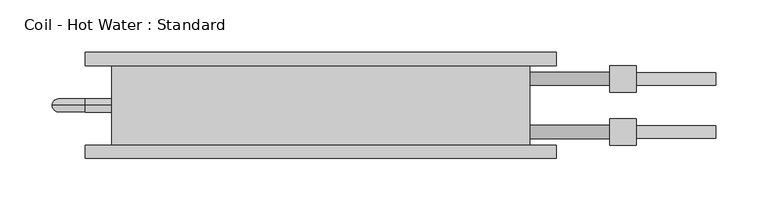
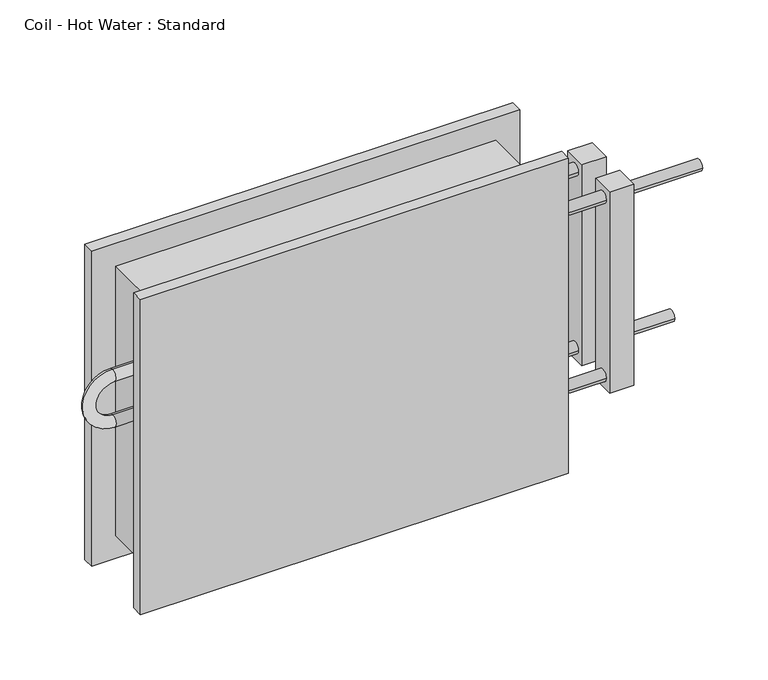
"""IFC4 building model written with IfcOpenShell, lengths in millimetres: proxy geometry, Coil - Hot Water : Standard."""

from ifc_helpers import new_model, si_unit, point, frame, origin, place, context, project, spatial, circle_curve, ellipse_curve, trimmed, source, transform, mapped, element, save
from ifc_brep_helpers import plane_surface, cylinder_surface, revolved_surface, advanced_brep


def coil_hot_water_standard_57d6a269(model_context):
    return source(origin(), model_context, "Body", "AdvancedBrep", [
        advanced_brep(
        [(-200.0, 76.2, 300.0), (-200.0, 0.0, 300.0), (200.0, 0.0, 300.0), (200.0, 76.2, 300.0), (200.0, 76.2, 0.0), (200.0, 0.0, 0.0), (-200.0, 0.0, 0.0), (-200.0, 76.2, 0.0), (-200.0, 38.1, 217.45), (-200.0, 38.1, 204.75), (-200.0, 38.1, 166.65), (-200.0, 38.1, 153.95), (200.0, 57.15, 249.2), (200.0, 69.85, 249.2), (200.0, 6.35, 50.8), (200.0, 19.05, 50.8), (200.0, 6.35, 249.2), (200.0, 19.05, 249.2), (200.0, 57.15, 50.8), (200.0, 69.85, 50.8), (225.4, 76.2, 325.4), (-225.4, 76.2, 325.4), (-225.4, 76.2, -25.4), (225.4, 76.2, -25.4), (225.4, 88.9, 325.4), (225.4, 88.9, -25.4), (-225.4, 88.9, -25.4), (-225.4, 88.9, 325.4), (377.8, 57.5, 50.8), (377.8, 69.5, 50.8), (377.8, 6.7, 249.2), (377.8, 18.7, 249.2), (301.6, 57.5, 50.8), (301.6, 69.5, 50.8), (301.6, 6.7, 249.2), (301.6, 18.7, 249.2), (225.4, -12.7, 325.4), (-225.4, -12.7, 325.4), (-225.4, -12.7, -25.4), (225.4, -12.7, -25.4), (225.4, 0.0, 325.4), (225.4, 0.0, -25.4), (-225.4, 0.0, -25.4), (-225.4, 0.0, 325.4), (-225.4, 38.1, 217.45), (-225.4, 38.1, 204.75), (-225.4, 38.1, 153.95), (-225.4, 38.1, 166.65), (276.2, 57.15, 249.2), (276.2, 69.85, 249.2), (276.2, 6.35, 50.8), (276.2, 19.05, 50.8), (276.2, 6.35, 249.2), (276.2, 19.05, 249.2), (276.2, 57.15, 50.8), (276.2, 69.85, 50.8), (301.6, 50.8, 261.9), (301.6, 50.8, 38.1), (301.6, 76.2, 38.1), (301.6, 76.2, 261.9), (301.6, 0.0, 261.9), (301.6, 0.0, 38.1), (301.6, 25.4, 38.1), (301.6, 25.4, 261.9), (276.2, 50.8, 261.9), (276.2, 76.2, 261.9), (276.2, 76.2, 38.1), (276.2, 50.8, 38.1), (276.2, 0.0, 261.9), (276.2, 25.4, 261.9), (276.2, 25.4, 38.1), (276.2, 0.0, 38.1)],
        [
            (0, 1),
            (1, 2),
            (2, 3),
            (3, 0),
            (4, 5),
            (5, 6),
            (6, 7),
            (7, 4),
            (0, 7),
            (6, 1),
            (8, 9, circle_curve(frame((-200.0, 38.1, 211.1), z_axis=(1.0, 0.0, 0.0), x_axis=(0.0, 0.0, -1.0)), 6.35)),
            (9, 8, circle_curve(frame((-200.0, 38.1, 211.1), z_axis=(1.0, 0.0, 0.0), x_axis=(0.0, 0.0, -1.0)), 6.35)),
            (10, 11, circle_curve(frame((-200.0, 38.1, 160.3), z_axis=(1.0, 0.0, 0.0), x_axis=(0.0, 0.0, 1.0)), 6.35)),
            (11, 10, circle_curve(frame((-200.0, 38.1, 160.3), z_axis=(1.0, 0.0, 0.0), x_axis=(0.0, 0.0, 1.0)), 6.35)),
            (2, 5),
            (4, 3),
            (12, 13, circle_curve(frame((200.0, 63.5, 249.2), z_axis=(-1.0, 0.0, 0.0), x_axis=(0.0, 1.0, 0.0)), 6.35)),
            (13, 12, circle_curve(frame((200.0, 63.5, 249.2), z_axis=(-1.0, 0.0, 0.0), x_axis=(0.0, 1.0, 0.0)), 6.35)),
            (14, 15, circle_curve(frame((200.0, 12.7, 50.8), z_axis=(-1.0, 0.0, 0.0), x_axis=(0.0, 1.0, 0.0)), 6.35)),
            (15, 14, circle_curve(frame((200.0, 12.7, 50.8), z_axis=(-1.0, 0.0, 0.0), x_axis=(0.0, 1.0, 0.0)), 6.35)),
            (16, 17, circle_curve(frame((200.0, 12.7, 249.2), z_axis=(-1.0, 0.0, 0.0), x_axis=(0.0, 1.0, 0.0)), 6.35)),
            (17, 16, circle_curve(frame((200.0, 12.7, 249.2), z_axis=(-1.0, 0.0, 0.0), x_axis=(0.0, 1.0, 0.0)), 6.35)),
            (18, 19, circle_curve(frame((200.0, 63.5, 50.8), z_axis=(-1.0, 0.0, 0.0), x_axis=(0.0, 1.0, 0.0)), 6.35)),
            (19, 18, circle_curve(frame((200.0, 63.5, 50.8), z_axis=(-1.0, 0.0, 0.0), x_axis=(0.0, 1.0, 0.0)), 6.35)),
            (20, 21),
            (21, 22),
            (22, 23),
            (23, 20),
            (24, 25),
            (25, 26),
            (26, 27),
            (27, 24),
            (20, 24),
            (27, 21),
            (26, 22),
            (25, 23),
            (28, 29, circle_curve(frame((377.8, 63.5, 50.8), z_axis=(1.0, 0.0, 0.0), x_axis=(0.0, 1.0, 0.0)), 6.0)),
            (29, 28, circle_curve(frame((377.8, 63.5, 50.8), z_axis=(1.0, 0.0, 0.0), x_axis=(0.0, 1.0, 0.0)), 6.0)),
            (30, 31, circle_curve(frame((377.8, 12.7, 249.2), z_axis=(1.0, 0.0, 0.0), x_axis=(0.0, 1.0, 0.0)), 6.0)),
            (31, 30, circle_curve(frame((377.8, 12.7, 249.2), z_axis=(1.0, 0.0, 0.0), x_axis=(0.0, 1.0, 0.0)), 6.0)),
            (28, 32),
            (32, 33, circle_curve(frame((301.6, 63.5, 50.8), z_axis=(1.0, 0.0, 0.0), x_axis=(0.0, 1.0, 0.0)), 6.0)),
            (33, 29),
            (33, 32, circle_curve(frame((301.6, 63.5, 50.8), z_axis=(1.0, 0.0, 0.0), x_axis=(0.0, 1.0, 0.0)), 6.0)),
            (30, 34),
            (34, 35, circle_curve(frame((301.6, 12.7, 249.2), z_axis=(1.0, 0.0, 0.0), x_axis=(0.0, 1.0, 0.0)), 6.0)),
            (35, 31),
            (35, 34, circle_curve(frame((301.6, 12.7, 249.2), z_axis=(1.0, 0.0, 0.0), x_axis=(0.0, 1.0, 0.0)), 6.0)),
            (36, 37),
            (37, 38),
            (38, 39),
            (39, 36),
            (40, 41),
            (41, 42),
            (42, 43),
            (43, 40),
            (36, 40),
            (43, 37),
            (42, 38),
            (41, 39),
            (8, 44),
            (44, 45, circle_curve(frame((-225.4, 38.1, 211.1), z_axis=(1.0, 0.0, 0.0), x_axis=(0.0, 0.0, -1.0)), 6.35)),
            (45, 9),
            (45, 44, circle_curve(frame((-225.4, 38.1, 211.1), z_axis=(1.0, 0.0, 0.0), x_axis=(0.0, 0.0, -1.0)), 6.35)),
            (44, 46, circle_curve(frame((-225.4, 38.1, 185.7), z_axis=(0.0, -1.0, 0.0), x_axis=(0.0, 0.0, 1.0)), 31.75)),
            (46, 47, circle_curve(frame((-225.4, 38.1, 160.3), z_axis=(-1.0, 0.0, 0.0), x_axis=(0.0, 0.0, 1.0)), 6.35)),
            (47, 45, circle_curve(frame((-225.4, 38.1, 185.7), z_axis=(0.0, 1.0, 0.0), x_axis=(0.0, 0.0, 1.0)), 19.05)),
            (47, 46, circle_curve(frame((-225.4, 38.1, 160.3), z_axis=(-1.0, 0.0, 0.0), x_axis=(0.0, 0.0, 1.0)), 6.35)),
            (46, 11),
            (10, 47),
            (12, 48),
            (48, 49, circle_curve(frame((276.2, 63.5, 249.2), z_axis=(-1.0, 0.0, 0.0), x_axis=(0.0, 1.0, 0.0)), 6.35)),
            (49, 13),
            (49, 48, circle_curve(frame((276.2, 63.5, 249.2), z_axis=(-1.0, 0.0, 0.0), x_axis=(0.0, 1.0, 0.0)), 6.35)),
            (14, 50),
            (50, 51, circle_curve(frame((276.2, 12.7, 50.8), z_axis=(-1.0, 0.0, 0.0), x_axis=(0.0, 1.0, 0.0)), 6.35)),
            (51, 15),
            (51, 50, circle_curve(frame((276.2, 12.7, 50.8), z_axis=(-1.0, 0.0, 0.0), x_axis=(0.0, 1.0, 0.0)), 6.35)),
            (16, 52),
            (52, 53, circle_curve(frame((276.2, 12.7, 249.2), z_axis=(-1.0, 0.0, 0.0), x_axis=(0.0, 1.0, 0.0)), 6.35)),
            (53, 17),
            (53, 52, circle_curve(frame((276.2, 12.7, 249.2), z_axis=(-1.0, 0.0, 0.0), x_axis=(0.0, 1.0, 0.0)), 6.35)),
            (18, 54),
            (54, 55, circle_curve(frame((276.2, 63.5, 50.8), z_axis=(-1.0, 0.0, 0.0), x_axis=(0.0, 1.0, 0.0)), 6.35)),
            (55, 19),
            (55, 54, circle_curve(frame((276.2, 63.5, 50.8), z_axis=(-1.0, 0.0, 0.0), x_axis=(0.0, 1.0, 0.0)), 6.35)),
            (56, 57),
            (57, 58),
            (58, 59),
            (59, 56),
            (60, 61),
            (61, 62),
            (62, 63),
            (63, 60),
            (64, 65),
            (65, 66),
            (66, 67),
            (67, 64),
            (68, 69),
            (69, 70),
            (70, 71),
            (71, 68),
            (56, 64),
            (67, 57),
            (66, 58),
            (65, 59),
            (60, 68),
            (71, 61),
            (70, 62),
            (69, 63),
        ],
        [
            plane_surface(frame((-200.0, 76.2, 300.0), z_axis=(0.0, 0.0, 1.0), x_axis=(-1.0, 0.0, 0.0))),
            plane_surface(frame((-200.0, 76.2, 0.0), z_axis=(0.0, 0.0, -1.0), x_axis=(1.0, 0.0, 0.0))),
            plane_surface(frame((-200.0, 76.2, 300.0), z_axis=(-1.0, 0.0, 0.0), x_axis=(0.0, 0.0, -1.0))),
            plane_surface(frame((200.0, 0.0, 300.0), z_axis=(1.0, 0.0, 0.0), x_axis=(0.0, 0.0, -1.0))),
            plane_surface(frame((-225.4, 76.2, 325.4), z_axis=(0.0, -1.0, 0.0), x_axis=(-1.0, 0.0, 0.0))),
            plane_surface(frame((-225.4, 88.9, 325.4), z_axis=(0.0, 1.0, 0.0), x_axis=(1.0, 0.0, 0.0))),
            plane_surface(frame((225.4, 76.2, 325.4), z_axis=(0.0, 0.0, 1.0), x_axis=(0.0, 1.0, 0.0))),
            plane_surface(frame((-225.4, 76.2, 325.4), z_axis=(-1.0, 0.0, 0.0), x_axis=(0.0, 1.0, 0.0))),
            plane_surface(frame((-225.4, 76.2, -25.4), z_axis=(0.0, 0.0, -1.0), x_axis=(0.0, 1.0, 0.0))),
            plane_surface(frame((225.4, 76.2, -25.4), z_axis=(1.0, 0.0, 0.0), x_axis=(0.0, 1.0, 0.0))),
            plane_surface(frame((377.8, 69.5, 50.8), z_axis=(1.0, 0.0, 0.0), x_axis=(0.0, 0.0, 1.0))),
            cylinder_surface(frame((301.6, 63.5, 50.8), z_axis=(1.0, 0.0, 0.0), x_axis=(0.0, 1.0, 0.0)), 6.0),
            cylinder_surface(frame((0.0, 12.7, 249.2), z_axis=(1.0, 0.0, 0.0), x_axis=(0.0, 1.0, 0.0)), 6.0),
            plane_surface(frame((-225.4, -12.7, 325.4), z_axis=(0.0, -1.0, 0.0), x_axis=(-1.0, 0.0, 0.0))),
            plane_surface(frame((-225.4, 0.0, 325.4), z_axis=(0.0, 1.0, 0.0), x_axis=(1.0, 0.0, 0.0))),
            plane_surface(frame((225.4, -12.7, 325.4), z_axis=(0.0, 0.0, 1.0), x_axis=(0.0, 1.0, 0.0))),
            plane_surface(frame((-225.4, -12.7, 325.4), z_axis=(-1.0, 0.0, 0.0), x_axis=(0.0, 1.0, 0.0))),
            plane_surface(frame((-225.4, -12.7, -25.4), z_axis=(0.0, 0.0, -1.0), x_axis=(0.0, 1.0, 0.0))),
            plane_surface(frame((225.4, -12.7, -25.4), z_axis=(1.0, 0.0, 0.0), x_axis=(0.0, 1.0, 0.0))),
            cylinder_surface(frame((-200.0, 38.1, 211.1), z_axis=(1.0, 0.0, 0.0), x_axis=(0.0, 0.0, -1.0)), 6.35),
            revolved_surface(trimmed(ellipse_curve(frame((-225.4, 38.1, 211.1), z_axis=(1.0, 0.0, 0.0), x_axis=(0.0, 0.0, -1.0)), 6.35, 6.35), [point((-225.4, 38.1, 217.45))], [point((-225.4, 38.1, 204.75))], True, "CARTESIAN"), (-225.4, 0.0, 185.7), (0.0, -1.0, 0.0)),
            revolved_surface(trimmed(ellipse_curve(frame((-225.4, 38.1, 211.1), z_axis=(1.0, 0.0, 0.0), x_axis=(0.0, 0.0, -1.0)), 6.35, 6.35), [point((-225.4, 38.1, 204.75))], [point((-225.4, 38.1, 217.45))], True, "CARTESIAN"), (-225.4, 0.0, 185.7), (0.0, -1.0, 0.0)),
            cylinder_surface(frame((-225.4, 38.1, 160.3), z_axis=(-1.0, 0.0, 0.0), x_axis=(0.0, 0.0, 1.0)), 6.35),
            cylinder_surface(frame((200.0, 63.5, 249.2), z_axis=(-1.0, 0.0, 0.0), x_axis=(0.0, 1.0, 0.0)), 6.35),
            cylinder_surface(frame((200.0, 12.7, 50.8), z_axis=(-1.0, 0.0, 0.0), x_axis=(0.0, 1.0, 0.0)), 6.35),
            cylinder_surface(frame((200.0, 12.7, 249.2), z_axis=(-1.0, 0.0, 0.0), x_axis=(0.0, 1.0, 0.0)), 6.35),
            cylinder_surface(frame((200.0, 63.5, 50.8), z_axis=(-1.0, 0.0, 0.0), x_axis=(0.0, 1.0, 0.0)), 6.35),
            plane_surface(frame((301.6, 50.8, 261.9), z_axis=(1.0, 0.0, 0.0), x_axis=(0.0, 0.0, -1.0))),
            plane_surface(frame((276.2, 50.8, 261.9), z_axis=(-1.0, 0.0, 0.0), x_axis=(0.0, 0.0, 1.0))),
            plane_surface(frame((301.6, 50.8, 261.9), z_axis=(0.0, -1.0, 0.0), x_axis=(-1.0, 0.0, 0.0))),
            plane_surface(frame((301.6, 50.8, 38.1), z_axis=(0.0, 0.0, -1.0), x_axis=(-1.0, 0.0, 0.0))),
            plane_surface(frame((301.6, 76.2, 38.1), z_axis=(0.0, 1.0, 0.0), x_axis=(-1.0, 0.0, 0.0))),
            plane_surface(frame((301.6, 76.2, 261.9), z_axis=(0.0, 0.0, 1.0), x_axis=(-1.0, 0.0, 0.0))),
            plane_surface(frame((301.6, 0.0, 261.9), z_axis=(0.0, -1.0, 0.0), x_axis=(-1.0, 0.0, 0.0))),
            plane_surface(frame((301.6, 0.0, 38.1), z_axis=(0.0, 0.0, -1.0), x_axis=(-1.0, 0.0, 0.0))),
            plane_surface(frame((301.6, 25.4, 38.1), z_axis=(0.0, 1.0, 0.0), x_axis=(-1.0, 0.0, 0.0))),
            plane_surface(frame((301.6, 25.4, 261.9), z_axis=(0.0, 0.0, 1.0), x_axis=(-1.0, 0.0, 0.0))),
        ],
        [
            (0, [[1, 2, 3, 4]]),
            (1, [[5, 6, 7, 8]]),
            (2, [[-1, 9, -7, 10], [11, 12], [13, 14]]),
            (3, [[-3, 15, -5, 16], [17, 18], [19, 20], [21, 22], [23, 24]]),
            (4, [[25, 26, 27, 28], [-4, -16, -8, -9]]),
            (5, [[29, 30, 31, 32]]),
            (6, [[-25, 33, -32, 34]]),
            (7, [[-26, -34, -31, 35]]),
            (8, [[-27, -35, -30, 36]]),
            (9, [[-28, -36, -29, -33]]),
            (10, [[37, 38]]),
            (10, [[39, 40]]),
            (11, [[-37, 41, 42, 43]]),
            (11, [[-38, -43, 44, -41]]),
            (12, [[-39, 45, 46, 47]]),
            (12, [[-40, -47, 48, -45]]),
            (13, [[49, 50, 51, 52]]),
            (14, [[53, 54, 55, 56], [-2, -10, -6, -15]]),
            (15, [[-49, 57, -56, 58]]),
            (16, [[-50, -58, -55, 59]]),
            (17, [[-51, -59, -54, 60]]),
            (18, [[-52, -60, -53, -57]]),
            (19, [[61, 62, 63, -11]]),
            (19, [[-61, -12, -63, 64]]),
            (20, [[-62, 65, 66, 67]]),
            (21, [[-64, -67, 68, -65]]),
            (22, [[-66, 69, -13, 70]]),
            (22, [[-68, -70, -14, -69]]),
            (23, [[71, 72, 73, -17]]),
            (23, [[-71, -18, -73, 74]]),
            (24, [[75, 76, 77, -19]]),
            (24, [[-75, -20, -77, 78]]),
            (25, [[79, 80, 81, -21]]),
            (25, [[-79, -22, -81, 82]]),
            (26, [[83, 84, 85, -23]]),
            (26, [[-83, -24, -85, 86]]),
            (27, [[87, 88, 89, 90], [-42, -44]]),
            (27, [[91, 92, 93, 94], [-46, -48]]),
            (28, [[95, 96, 97, 98], [-72, -74], [-84, -86]]),
            (28, [[99, 100, 101, 102], [-76, -78], [-80, -82]]),
            (29, [[-87, 103, -98, 104]]),
            (30, [[-88, -104, -97, 105]]),
            (31, [[-89, -105, -96, 106]]),
            (32, [[-90, -106, -95, -103]]),
            (33, [[-91, 107, -102, 108]]),
            (34, [[-92, -108, -101, 109]]),
            (35, [[-93, -109, -100, 110]]),
            (36, [[-94, -110, -99, -107]]),
        ],
    ),
    ])


if __name__ == "__main__":
    model = new_model("IFC4")
    model_context = context("Model", 3, world=origin())
    ifc_project = project(units=[si_unit("LENGTHUNIT", "METRE", prefix="MILLI")], contexts=[model_context])
    site = spatial("IfcSite", under=ifc_project)
    building = spatial("IfcBuilding", under=site)
    placement = place(None, origin())
    coil_hot_water_standard_shape = coil_hot_water_standard_57d6a269(model_context)
    element("IfcBuildingElementProxy", 1, Name="Coil - Hot Water : Standard", ObjectType="Coil - Hot Water : Standard", at=placement, inside=building, context=model_context, shape_type="MappedRepresentation", body=[
        mapped(coil_hot_water_standard_shape, transform((0.0, 0.0, 0.0), x_axis=(1.0, 0.0, 0.0), y_axis=(0.0, 1.0, 0.0), z_axis=(0.0, 0.0, 1.0))),
    ])
    save(model, "model.ifc")

# Revit data of these elements
# Type "Coil - Hot Water : Standard"
#   Duct Width [instance default] = 16"
#   Duct Height [instance default] = 12"
#   Coil Length [instance default] = 1' - 10 1/4"
#   Water Radius = 0.23622"
#   Water Pressure Drop [instance default] = 0.00 psi
#   Water Flow [instance default] = 0 GPM
#   Water Diameter = 0.47244"
#   Air Pressure Drop [instance default] = 0.03 in-wg
#   Air Flow [instance default] = 500 CFM
#   Coil Material = none
#   Assembly Code = ""
# Element 1 (IfcBuildingElementProxy, "Coil - Hot Water : Standard")
#   Duct Width = 15.74803"
#   Duct Height = 11.81102"
#   Coil Length = 1' - 9.99803"
